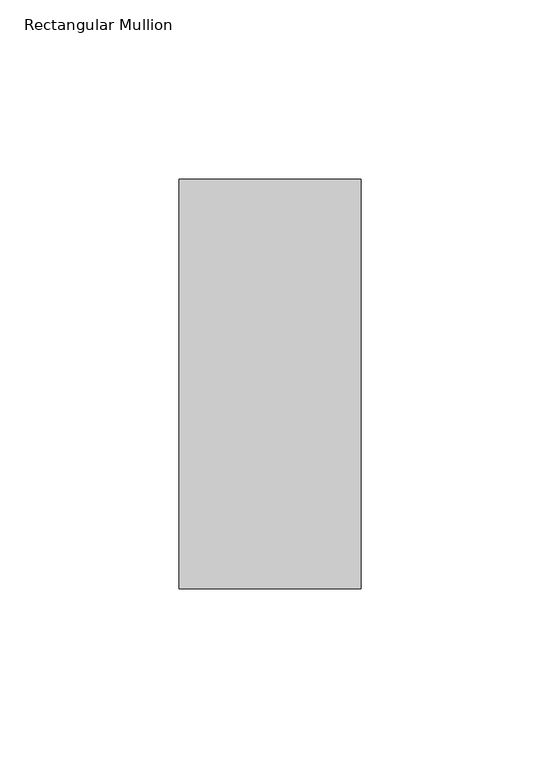
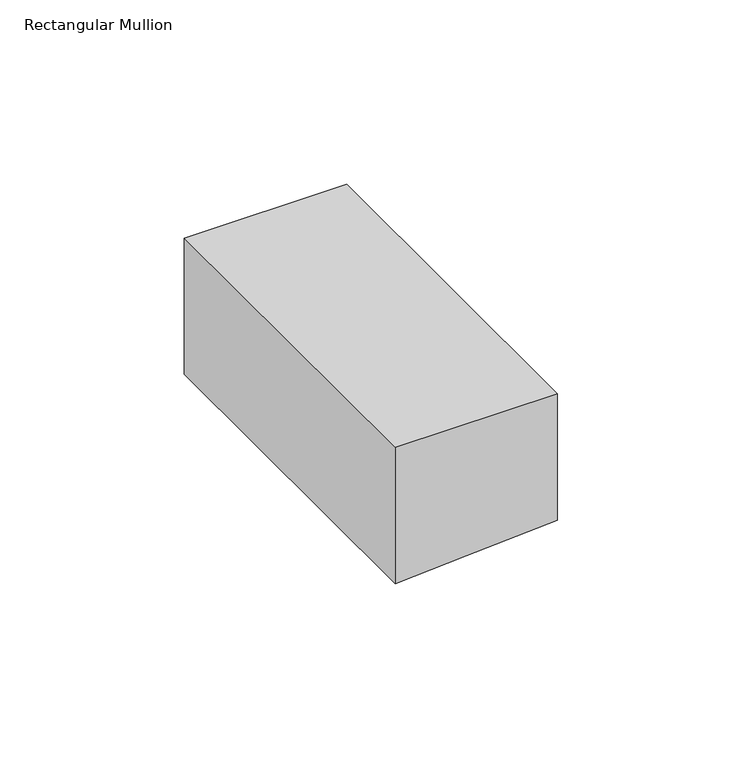
"""IFC4 building model written with IfcOpenShell, lengths in millimetres: member geometry, Rectangular Mullion : KAWNEER TRIFAB VERSAGLAZE 451T - CLEAR ANODIZED ALUM. - BACK GLAZED."""

from ifc_helpers import new_model, si_unit, frame, origin, place, context, project, spatial, polyline, outline, extrude, source, transform, mapped, element, save


def rectangular_mullion_925f85da(model_context):
    return source(origin(), model_context, "Body", "SweptSolid", [
        extrude(outline(polyline([(0.0, 25.4), (0.0, -25.4), (-45.0831344, -25.4), (-43.6936855, -3.1688169), (-41.9081344, 25.4), (0.0, 25.4)])), frame((0.0, -57.15, 0.0), z_axis=(0.0, 1.0, 0.0), x_axis=(0.0, 0.0, 1.0)), (0.0, 0.0, 1.0), 114.3),
    ])


if __name__ == "__main__":
    model = new_model("IFC4")
    model_context = context("Model", 3, world=origin())
    ifc_project = project(units=[si_unit("LENGTHUNIT", "METRE", prefix="MILLI")], contexts=[model_context])
    site = spatial("IfcSite", under=ifc_project)
    building = spatial("IfcBuilding", under=site)
    placement = place(None, origin())
    rectangular_mullion_shape = rectangular_mullion_925f85da(model_context)
    element("IfcMember", 1, ObjectType="Rectangular Mullion : KAWNEER TRIFAB VERSAGLAZE 451T - CLEAR ANODIZED ALUM. - BACK GLAZED", at=placement, inside=building, context=model_context, shape_type="MappedRepresentation", body=[
        mapped(rectangular_mullion_shape, transform((0.0, 0.0, 0.0), x_axis=(1.0, 0.0, 0.0), y_axis=(0.0, 1.0, 0.0), z_axis=(0.0, 0.0, 1.0))),
    ])
    save(model, "model.ifc")

# Revit data of these elements
# Type "Rectangular Mullion : KAWNEER TRIFAB VERSAGLAZE 451T - CLEAR ANODIZED ALUM. - BACK GLAZED"
#   built-in parameter 1007304 = 0.375 (stored number, unit not read)
#   built-in parameter 1007301 = 0.0833333 (stored number, unit not read)
#   built-in parameter 1007300 = 0.0833333 (stored number, unit not read)
# Element 1 (IfcMember, "Rectangular Mullion : KAWNEER TRIFAB VERSAGLAZE 451T - CLEAR ANODIZED ALUM. - BACK GLAZED")
#   Materials on its faces: "KAWNEER TRIFAB VERSAGLAZE 451T - CLEAR ANODIZED ALUM. - BACK GLAZED"
# Materials
#   "KAWNEER TRIFAB VERSAGLAZE 451T - CLEAR ANODIZED ALUM. - BACK GLAZED": class "Metal", colour RGB 244 244 244, transparency 0, Description = "Aluminum 6061", Cost = 0
